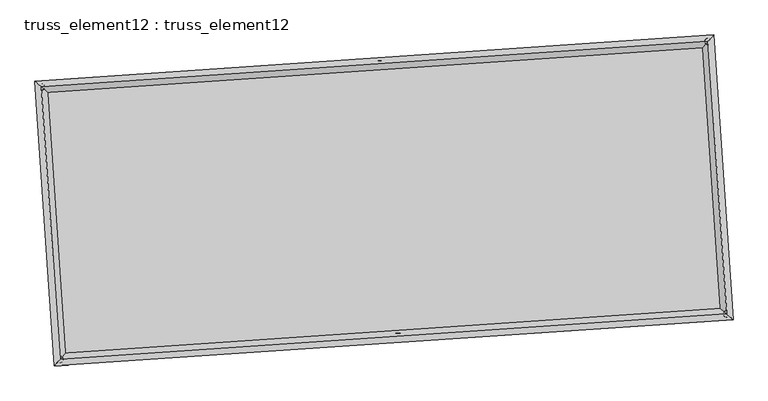
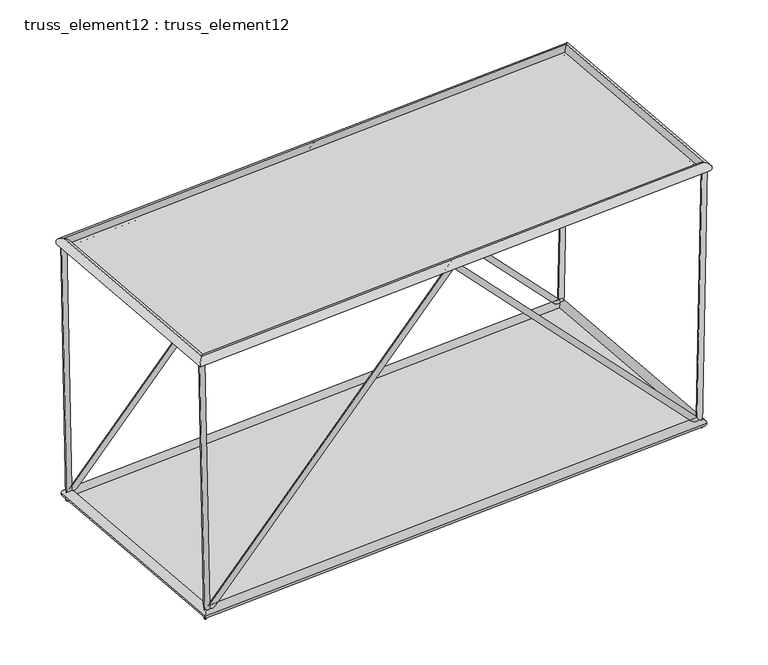
"""IFC4 building model written with IfcOpenShell, lengths in millimetres: plate geometry, truss_element12 : truss_element12."""

import ifcopenshell
import ifcopenshell.guid

model = None  # the IFC model being written
_history = None  # IfcOwnerHistory: only IFC2X3 demands one
_inside = {}  # id of a spatial element -> (the spatial element, [elements in it])
_under = {}  # id of a project, library or spatial element -> (it, [spatial elements below it])
_declared = {}  # id of a project -> (the project, [libraries it declares])
_typed = {}  # id of a type object -> (the type object, [elements of that type])
_made_of = {}  # id of a material, layer set ... -> (it, [elements and type objects made of it])


def new_model(schema):
    """Start an empty IFC model of exactly this schema.

    Asked for "IFC4X3", IfcOpenShell would pick the latest addendum, in which some entities
    have other attributes; the version numbers below select the first issue.
    IFC2X3 requires an IfcOwnerHistory on every rooted entity: one is made here for all.
    """
    global model, _history
    if schema == "IFC4X3":
        model = ifcopenshell.file(schema_version=(4, 3, 0, 0))
    else:
        model = ifcopenshell.file(schema=schema)
    _inside.clear()
    _under.clear()
    _declared.clear()
    _typed.clear()
    _made_of.clear()
    _history = None
    if model.schema == "IFC2X3":
        org = make("IfcOrganization", Name="unknown")
        user = make(
            "IfcPersonAndOrganization",
            ThePerson=make("IfcPerson", FamilyName="unknown"),
            TheOrganization=org,
        )
        app = make(
            "IfcApplication",
            ApplicationDeveloper=org,
            Version="unknown",
            ApplicationFullName="unknown",
            ApplicationIdentifier="unknown",
        )
        _history = make(
            "IfcOwnerHistory",
            OwningUser=user,
            OwningApplication=app,
            ChangeAction="ADDED",
            CreationDate=0,
        )
    return model


def make(cls, **values):
    """One entity of the class cls with the attributes given. An attribute that is None is left unset."""
    return model.create_entity(
        cls, **{name: value for name, value in values.items() if value is not None}
    )


def rooted(cls, **values):
    """An entity with a GlobalId (a new one), such as an element, a storey or a relation."""
    return make(cls, GlobalId=ifcopenshell.guid.new(), OwnerHistory=_history, **values)


def si_unit(unit_type, name, prefix=None):
    """IfcSIUnit, for example si_unit("LENGTHUNIT", "METRE", prefix="MILLI")."""
    return make("IfcSIUnit", UnitType=unit_type, Prefix=prefix, Name=name)


def assignment(units):
    """IfcUnitAssignment: the units of a project."""
    return None if units is None else make("IfcUnitAssignment", Units=units)


def point(xyz):
    """IfcCartesianPoint."""
    return None if xyz is None else make("IfcCartesianPoint", Coordinates=xyz)


def direction(xyz):
    """IfcDirection."""
    return None if xyz is None else make("IfcDirection", DirectionRatios=xyz)


def frame(location, z_axis=None, x_axis=None):
    """IfcAxis2Placement3D, a coordinate frame: its origin and axes. An axis left out is left unset."""
    return make(
        "IfcAxis2Placement3D",
        Location=point(location),
        Axis=direction(z_axis),
        RefDirection=direction(x_axis),
    )


def origin():
    """The frame at (0, 0, 0) with its axes left unset."""
    return frame((0.0, 0.0, 0.0))


def origin_with_axes():
    """The frame at (0, 0, 0) with the z axis (0, 0, 1) and the x axis (1, 0, 0) written out."""
    return frame((0.0, 0.0, 0.0), z_axis=(0.0, 0.0, 1.0), x_axis=(1.0, 0.0, 0.0))


def place(relative_to, where):
    """IfcLocalPlacement: puts the frame where relative to a parent placement (None: the world)."""
    return make(
        "IfcLocalPlacement", PlacementRelTo=relative_to, RelativePlacement=where
    )


def context(
    kind, dimensions, precision=None, world=None, true_north=None, identifier=None
):
    """IfcGeometricRepresentationContext, for example the 3D "Model" context."""
    return make(
        "IfcGeometricRepresentationContext",
        ContextIdentifier=identifier,
        ContextType=kind,
        CoordinateSpaceDimension=dimensions,
        Precision=precision,
        WorldCoordinateSystem=world,
        TrueNorth=true_north,
    )


def project(units=None, contexts=None):
    """IfcProject with its units and contexts."""
    return rooted(
        "IfcProject",
        Name="project",
        RepresentationContexts=contexts,
        UnitsInContext=assignment(units),
    )


def spatial(cls, under=None, at=None, **own):
    """A site, building, storey or space (cls), placed at a placement, below another one or the project."""
    s = rooted(cls, ObjectPlacement=at, **own)
    if under is not None:
        _under.setdefault(under.id(), (under, []))[1].append(s)
    return s


def polyline(points):
    """IfcPolyline through the points."""
    return make("IfcPolyline", Points=[point(p) for p in points])


def circle_curve(where, radius):
    """IfcCircle in the frame where."""
    return make("IfcCircle", Position=where, Radius=radius)


def ellipse_curve(where, semi_axis1, semi_axis2):
    """IfcEllipse in the frame where."""
    return make(
        "IfcEllipse", Position=where, SemiAxis1=semi_axis1, SemiAxis2=semi_axis2
    )


def outline(outer, holes=None, kind="AREA"):
    """IfcArbitraryClosedProfileDef: a profile drawn as a closed curve; with holes, ...WithVoids."""
    if holes is None:
        return make("IfcArbitraryClosedProfileDef", ProfileType=kind, OuterCurve=outer)
    return make(
        "IfcArbitraryProfileDefWithVoids",
        ProfileType=kind,
        OuterCurve=outer,
        InnerCurves=holes,
    )


def extrude(swept, where, along, depth):
    """IfcExtrudedAreaSolid: the profile swept, set in the frame where, extruded along a direction by depth."""
    return make(
        "IfcExtrudedAreaSolid",
        SweptArea=swept,
        Position=where,
        ExtrudedDirection=direction(along),
        Depth=depth,
    )


def shape(context_of_items, identifier, shape_type, items):
    """IfcShapeRepresentation: the items that make up one representation, for example the "Body"."""
    return make(
        "IfcShapeRepresentation",
        ContextOfItems=context_of_items,
        RepresentationIdentifier=identifier,
        RepresentationType=shape_type,
        Items=items,
    )


def source(mapping_origin, context_of_items, identifier, shape_type, items):
    """IfcRepresentationMap: a shape defined once, which mapped items show again and again."""
    return make(
        "IfcRepresentationMap",
        MappingOrigin=mapping_origin,
        MappedRepresentation=shape(context_of_items, identifier, shape_type, items),
    )


def transform(
    local_origin,
    x_axis=None,
    y_axis=None,
    z_axis=None,
    scale=None,
    scale2=None,
    scale3=None,
    uniform=True,
):
    """IfcCartesianTransformationOperator3D, or its non-uniform kind. x_axis, y_axis, z_axis: its Axis1, 2, 3."""
    if uniform:
        return make(
            "IfcCartesianTransformationOperator3D",
            Axis1=direction(x_axis),
            Axis2=direction(y_axis),
            LocalOrigin=point(local_origin),
            Scale=scale,
            Axis3=direction(z_axis),
        )
    return make(
        "IfcCartesianTransformationOperator3DnonUniform",
        Axis1=direction(x_axis),
        Axis2=direction(y_axis),
        LocalOrigin=point(local_origin),
        Scale=scale,
        Axis3=direction(z_axis),
        Scale2=scale2,
        Scale3=scale3,
    )


def mapped(mapping_source, mapping_target):
    """IfcMappedItem: shows the shape of a source again, moved by a transform."""
    return make(
        "IfcMappedItem", MappingSource=mapping_source, MappingTarget=mapping_target
    )


def made_of(thing, what):
    """Note that an element or type object is made of a material, layer set ...; save() writes the relation."""
    if what is not None:
        _made_of.setdefault(what.id(), (what, []))[1].append(thing)
    return thing


def element(
    cls,
    number,
    at=None,
    inside=None,
    cuts=None,
    type_object=None,
    material=None,
    context=None,
    identifier="Body",
    shape_type=None,
    held_by="IfcProductDefinitionShape",
    body=None,
    shapes=None,
    **own,
):
    """One element of the class cls, such as IfcWall. Its Tag is "e" and its number.

    at: its placement. inside: the storey or other place that contains it. cuts: it is an
    opening in that element (IfcRelVoidsElement). A single representation is given by context,
    identifier, shape_type and body (its items); several are given by shapes. held_by: the class
    of the entity that holds the representations. save() writes the other relations.
    """
    e = rooted(cls, Tag="e%d" % number, ObjectPlacement=at, **own)
    if body is not None:
        shapes = [shape(context, identifier, shape_type, body)]
    if shapes is not None:
        e.Representation = make(held_by, Representations=shapes)
    if inside is not None:
        _inside.setdefault(inside.id(), (inside, []))[1].append(e)
    if cuts is not None:
        rooted(
            "IfcRelVoidsElement", RelatingBuildingElement=cuts, RelatedOpeningElement=e
        )
    if type_object is not None:
        _typed.setdefault(type_object.id(), (type_object, []))[1].append(e)
    return made_of(e, material)


def aggregate(whole, parts):
    """IfcRelAggregates: a whole, such as a stair, and the parts it consists of."""
    return rooted("IfcRelAggregates", RelatingObject=whole, RelatedObjects=parts)


def save(model, path):
    """Write the relations noted so far, then the file.

    IfcRelAggregates (storeys below a building ...), IfcRelContainedInSpatialStructure (elements
    in a storey), IfcRelDefinesByType, IfcRelAssociatesMaterial and IfcRelDeclares: one each for
    every whole, place, type object, material and project.
    """
    for whole, parts in _under.values():
        aggregate(whole, parts)
    for where, things in _inside.values():
        rooted(
            "IfcRelContainedInSpatialStructure",
            RelatedElements=things,
            RelatingStructure=where,
        )
    for kind, things in _typed.values():
        rooted("IfcRelDefinesByType", RelatedObjects=things, RelatingType=kind)
    for what, things in _made_of.values():
        rooted("IfcRelAssociatesMaterial", RelatedObjects=things, RelatingMaterial=what)
    for by, libraries in _declared.values():
        rooted("IfcRelDeclares", RelatingContext=by, RelatedDefinitions=libraries)
    model.write(path)


def plane_surface(at):
    """IfcPlane: the flat surface through the origin of the frame at, square to its z axis."""
    return make("IfcPlane", Position=at)


def cylinder_surface(at, radius):
    """IfcCylindricalSurface: all points at the distance radius from the z axis of the frame at."""
    return make("IfcCylindricalSurface", Position=at, Radius=radius)


def advanced_brep(points, edges, surfaces, faces):
    """IfcAdvancedBrep: a solid bounded by faces that lie on surfaces and meet in shared edges.

    An edge is (start, end): straight between two places in points (the first is 0);
    or (start, end, curve); or (start, end, curve, False) where it runs against its curve.
    A face is (place in surfaces, loops), or (place, loops, False) where it looks against
    its surface's normal. A loop lists edges by number (the first is 1), with a minus sign
    where the edge is run from its end to its start. The first loop is the outer one.
    """
    corners = [point(p) for p in points]
    vertices = [make("IfcVertexPoint", VertexGeometry=c) for c in corners]
    made = []
    for start, end, *more in edges:
        made.append(
            make(
                "IfcEdgeCurve",
                EdgeStart=vertices[start],
                EdgeEnd=vertices[end],
                EdgeGeometry=more[0] if more else make("IfcPolyline", Points=[corners[start], corners[end]]),
                SameSense=more[1] if len(more) > 1 else True,
            )
        )
    hull = []
    for where, loops, *sense in faces:
        bounds = []
        for j, loop in enumerate(loops):
            ring = [make("IfcOrientedEdge", EdgeElement=made[abs(k) - 1], Orientation=k > 0) for k in loop]
            bounds.append(
                make(
                    "IfcFaceOuterBound" if j == 0 else "IfcFaceBound",
                    Bound=make("IfcEdgeLoop", EdgeList=ring),
                    Orientation=True,
                )
            )
        hull.append(make("IfcAdvancedFace", Bounds=bounds, FaceSurface=surfaces[where], SameSense=sense[0] if sense else True))
    return make("IfcAdvancedBrep", Outer=make("IfcClosedShell", CfsFaces=hull))


def truss_element12_truss_element12_cebb5c17(model_context):
    return source(origin(), model_context, "Body", "SolidModel", [
        advanced_brep(
        [(-3767.1671851, 2269.2535853, 4999.9725392), (-3866.2496537, 2255.8937932, 4997.9279448), (-3667.4174306, 2276.0551419, 121.5871098), (-3761.5694522, 2263.0315382, -121.5871098), (1064.3618326, 2598.6971827, 5071.0530248), (1064.8004406, 2592.1233545, 4926.8210996), (5794.886864, 2921.2537021, 121.578348), (5889.874113, 2921.1267864, -121.578348), (5895.881521, 2928.1401439, 4999.9589337), (5995.8598643, 2928.3535519, 4997.8888311)],
        [
            (0, 1, circle_curve(frame((-3816.7084194, 2262.5736893, 4998.950242), z_axis=(-0.020442995593720103, -0.0013939301584342944, 0.9997900484050983), x_axis=(-0.13359837212382125, 0.9910346373676144, -0.001350001298501484)), 50.0)),
            (1, 0, circle_curve(frame((-3816.7084194, 2262.5736893, 4998.950242), z_axis=(-0.020442995593720103, -0.0013939301584342944, 0.9997900484050983), x_axis=(-0.13359837212382125, 0.9910346373676144, -0.001350001298501484)), 50.0)),
            (0, 2),
            (2, 3, ellipse_curve(frame((-3714.4934414, 2269.54334, 0.0), z_axis=(-0.9295196526265942, -0.06338041167761023, 0.3632852031070248), x_axis=(0.36244361517956775, 0.024713652341926906, 0.9316779814954776)), 130.7875297, 50.0)),
            (3, 1),
            (3, 2, ellipse_curve(frame((-3714.4934414, 2269.54334, 0.0), z_axis=(-0.9295196526265942, -0.06338041167761023, 0.3632852031070248), x_axis=(0.36244361517956775, 0.024713652341926906, 0.9316779814954776)), 130.7875297, 50.0)),
            (2, 4),
            (4, 5, ellipse_curve(frame((1064.5811366, 2595.4102686, 4998.9370622), z_axis=(-0.9976833938584647, -0.06802823807757291, 6.66567062485209e-05), x_axis=(-6.650228906135178e-05, -4.534538292208103e-06, -0.9999999977784416)), 72.2729929, 50.0)),
            (5, 3),
            (5, 4, ellipse_curve(frame((1064.5811366, 2595.4102686, 4998.9370622), z_axis=(-0.9976833938584647, -0.06802823807757291, 6.66567062485209e-05), x_axis=(-6.650228906135178e-05, -4.534538292208103e-06, -0.9999999977784416)), 72.2729929, 50.0)),
            (4, 6),
            (6, 7, ellipse_curve(frame((5842.3804885, 2921.1902443, 0.0), z_axis=(-0.9295901312719009, -0.06338521734851923, -0.36310398243970066), x_axis=(-0.3622628143287533, -0.024701324219198302, 0.9317486237910036)), 130.7681897, 50.0)),
            (7, 5),
            (7, 6, ellipse_curve(frame((5842.3804885, 2921.1902443, 0.0), z_axis=(-0.9295901312719009, -0.06338521734851923, -0.36310398243970066), x_axis=(-0.3622628143287533, -0.024701324219198302, 0.9317486237910036)), 130.7681897, 50.0)),
            (8, 9, circle_curve(frame((5945.8706927, 2928.2468479, 4998.9238824), z_axis=(0.020698040829792947, 0.0014113207235643172, 0.9997847764792299), x_axis=(-0.0021628361331172694, 0.999996726933573, -0.0013668438105636789)), 50.0)),
            (9, 8, circle_curve(frame((5945.8706927, 2928.2468479, 4998.9238824), z_axis=(0.020698040829792947, 0.0014113207235643172, 0.9997847764792299), x_axis=(-0.0021628361331172694, 0.999996726933573, -0.0013668438105636789)), 50.0)),
            (6, 8),
            (9, 7),
        ],
        [
            plane_surface(frame((-3816.7084194, 2312.5736407, 4999.0199531), z_axis=(-0.020442995593718667, -0.0013939301584386158, 0.9997900484050983), x_axis=(0.9997910201292846, -2.8502064444602113e-05, 0.020442975724613167))),
            cylinder_surface(frame((-3816.7084194, 2262.5736893, 4998.950242), z_axis=(-0.0204429955937201, -0.0013939301584342942, 0.9997900484050981), x_axis=(-0.13359837212382125, 0.9910346373676144, -0.001350001298501484)), 50.0),
            cylinder_surface(frame((-3714.4934414, 2269.54334, 0.0), z_axis=(-0.6902666987206841, -0.047066662236389376, -0.7220225854799657), x_axis=(-0.020420628738629147, 0.9987517974601704, -0.04558338504321424)), 50.0),
            cylinder_surface(frame((1064.5811366, 2595.4102686, 4998.9370622), z_axis=(-0.6901706602776501, -0.0470601137400352, 0.7221148145459193), x_axis=(-0.11534629536258453, 0.9922791770993238, -0.04557704291873413)), 50.0),
            plane_surface(frame((5945.8706927, 2878.2468977, 4998.9944636), z_axis=(0.02069804082979222, 0.0014113207235603308, 0.9997847764792298), x_axis=(0.999785772606216, -2.921783322129555e-05, -0.020698020207497326))),
            cylinder_surface(frame((5842.3804885, 2921.1902443, 0.0), z_axis=(-0.020698040829792947, -0.0014113207235643172, -0.9997847764792299), x_axis=(-0.0021628361331172694, 0.999996726933573, -0.0013668438105636789)), 50.0),
        ],
        [
            (0, [[1, 2]]),
            (1, [[-1, 3, 4, 5]]),
            (1, [[-2, -5, 6, -3]]),
            (2, [[-4, 7, 8, 9]]),
            (2, [[-6, -9, 10, -7]]),
            (3, [[-8, 11, 12, 13]]),
            (3, [[-10, -13, 14, -11]]),
            (4, [[15, 16]]),
            (5, [[-12, 17, -16, 18]]),
            (5, [[-14, -18, -15, -17]]),
        ],
    ),
        advanced_brep(
        [(-3495.0542322, -1721.479999, 4999.9725392), (-3594.1367008, -1734.8397911, 4997.9279448), (-3395.3044777, -1714.6784424, 121.5871098), (-3489.4564993, -1727.7020461, -121.5871098), (1336.4747855, -1392.0364016, 5071.0530248), (1336.9133936, -1398.6102298, 4926.8210996), (6066.9998169, -1069.4798822, 121.578348), (6161.9870659, -1069.6067979, -121.578348), (6167.9944739, -1062.5934404, 4999.9589337), (6267.9728172, -1062.3800324, 4997.8888311)],
        [
            (0, 1, circle_curve(frame((-3544.5954665, -1728.159895, 4998.950242), z_axis=(-0.0204429955937201, -0.001393930158434303, 0.9997900484050983), x_axis=(-0.1335983721238217, 0.9910346373676143, -0.001350001298501484)), 50.0)),
            (1, 0, circle_curve(frame((-3544.5954665, -1728.159895, 4998.950242), z_axis=(-0.0204429955937201, -0.001393930158434303, 0.9997900484050983), x_axis=(-0.1335983721238217, 0.9910346373676143, -0.001350001298501484)), 50.0)),
            (0, 2),
            (2, 3, ellipse_curve(frame((-3442.3804885, -1721.1902443, 0.0), z_axis=(-0.9295196526265942, -0.06338041167761047, 0.3632852031070248), x_axis=(0.36244361517956775, 0.024713652341926996, 0.9316779814954776)), 130.7875297, 50.0)),
            (3, 1),
            (3, 2, ellipse_curve(frame((-3442.3804885, -1721.1902443, 0.0), z_axis=(-0.9295196526265942, -0.06338041167761047, 0.3632852031070248), x_axis=(0.36244361517956775, 0.024713652341926996, 0.9316779814954776)), 130.7875297, 50.0)),
            (2, 4),
            (4, 5, ellipse_curve(frame((1336.6940895, -1395.3233157, 4998.9370622), z_axis=(-0.9976833938584648, -0.06802823807757319, 6.66567062488419e-05), x_axis=(-6.650228906135175e-05, -4.534538292198492e-06, -0.9999999977784417)), 72.2729929, 50.0)),
            (5, 3),
            (5, 4, ellipse_curve(frame((1336.6940895, -1395.3233157, 4998.9370622), z_axis=(-0.9976833938584648, -0.06802823807757319, 6.66567062488419e-05), x_axis=(-6.650228906135175e-05, -4.534538292198492e-06, -0.9999999977784417)), 72.2729929, 50.0)),
            (4, 6),
            (6, 7, ellipse_curve(frame((6114.4934414, -1069.54334, 0.0), z_axis=(-0.9295901312719014, -0.06338521734851954, -0.3631039824397004), x_axis=(-0.36226281432875257, -0.02470132421919832, 0.931748623791004)), 130.7681897, 50.0)),
            (7, 5),
            (7, 6, ellipse_curve(frame((6114.4934414, -1069.54334, 0.0), z_axis=(-0.9295901312719014, -0.06338521734851954, -0.3631039824397004), x_axis=(-0.36226281432875257, -0.02470132421919832, 0.931748623791004)), 130.7681897, 50.0)),
            (8, 9, circle_curve(frame((6217.9836456, -1062.4867364, 4998.9238824), z_axis=(0.020698040829793325, 0.0014113207235643879, 0.9997847764792299), x_axis=(-0.0021628361331172976, 0.999996726933573, -0.0013668438105637482)), 50.0)),
            (9, 8, circle_curve(frame((6217.9836456, -1062.4867364, 4998.9238824), z_axis=(0.020698040829793325, 0.0014113207235643879, 0.9997847764792299), x_axis=(-0.0021628361331172976, 0.999996726933573, -0.0013668438105637482)), 50.0)),
            (6, 8),
            (9, 7),
        ],
        [
            plane_surface(frame((-3544.5954665, -1678.1599436, 4999.0199531), z_axis=(-0.020442995593718667, -0.0013939301584386119, 0.9997900484050983), x_axis=(0.9997910201292846, -2.8502064444602113e-05, 0.020442975724613167))),
            cylinder_surface(frame((-3544.5954665, -1728.159895, 4998.950242), z_axis=(-0.020442995593720096, -0.0013939301584343028, 0.9997900484050981), x_axis=(-0.1335983721238217, 0.9910346373676143, -0.001350001298501484)), 50.0),
            cylinder_surface(frame((-3442.3804885, -1721.1902443, 0.0), z_axis=(-0.6902666987206841, -0.04706666223638955, -0.7220225854799657), x_axis=(-0.020420628738629217, 0.9987517974601704, -0.04558338504321442)), 50.0),
            cylinder_surface(frame((1336.6940895, -1395.3233157, 4998.9370622), z_axis=(-0.6901706602776495, -0.04706011374003534, 0.7221148145459199), x_axis=(-0.11534629536258498, 0.9922791770993238, -0.04557704291873424)), 50.0),
            plane_surface(frame((6217.9836456, -1112.4866866, 4998.9944636), z_axis=(0.020698040829792222, 0.0014113207235603214, 0.9997847764792299), x_axis=(0.999785772606216, -2.9217833220407372e-05, -0.020698020207497326))),
            cylinder_surface(frame((6114.4934414, -1069.54334, 0.0), z_axis=(-0.020698040829793325, -0.0014113207235643879, -0.9997847764792299), x_axis=(-0.0021628361331172976, 0.999996726933573, -0.0013668438105637482)), 50.0),
        ],
        [
            (0, [[1, 2]]),
            (1, [[-1, 3, 4, 5]]),
            (1, [[-2, -5, 6, -3]]),
            (2, [[-4, 7, 8, 9]]),
            (2, [[-6, -9, 10, -7]]),
            (3, [[-8, 11, 12, 13]]),
            (3, [[-10, -13, 14, -11]]),
            (4, [[15, 16]]),
            (5, [[-12, 17, -16, 18]]),
            (5, [[-14, -18, -15, -17]]),
        ],
    ),
        advanced_brep(
        [(-3544.602327, -1728.1674988, 4908.9502423), (-3544.5886059, -1728.1522913, 5088.9502417), (-3816.7005902, 2262.5670871, 5088.9502417), (-3816.7162486, 2262.5802914, 4908.9502423), (5945.8643159, 2928.2392771, 5088.9238821), (5945.8770694, 2928.2544187, 4908.9238827), (6217.9763001, -1062.4801013, 5088.9238821), (6217.990991, -1062.4933716, 4908.9238827)],
        [
            (0, 1, ellipse_curve(frame((-3544.5954665, -1728.159895, 4998.950242), z_axis=(-0.7535719234028931, 0.6573654662782613, 1.9048135841045667e-06), x_axis=(-0.6573654662755273, -0.7535719234052781, 1.9048135841050712e-06)), 127.2792206, 90.0)),
            (1, 2),
            (2, 3, ellipse_curve(frame((-3816.7084194, 2262.5736893, 4998.950242), z_axis=(-0.657365466275527, -0.7535719234052783, 1.904813584105534e-06), x_axis=(0.7535719234028931, -0.6573654662782611, -1.9048135841050305e-06)), 127.2792206, 90.0)),
            (3, 0),
            (1, 0, ellipse_curve(frame((-3544.5954665, -1728.159895, 4998.950242), z_axis=(-0.7535719234028931, 0.6573654662782613, 1.9048135841045667e-06), x_axis=(-0.6573654662755273, -0.7535719234052781, 1.9048135841050712e-06)), 127.2792206, 90.0)),
            (3, 2, ellipse_curve(frame((-3816.7084194, 2262.5736893, 4998.950242), z_axis=(-0.657365466275527, -0.7535719234052783, 1.904813584105534e-06), x_axis=(0.7535719234028931, -0.6573654662782611, -1.9048135841050305e-06)), 127.2792206, 90.0)),
            (2, 4),
            (4, 5, ellipse_curve(frame((5945.8706927, 2928.2468479, 4998.9238824), z_axis=(-0.7535719234028928, 0.6573654662782618, 1.9048135841054962e-06), x_axis=(-0.6573654662755274, -0.7535719234052779, 1.9048135841050684e-06)), 127.2792206, 90.0)),
            (5, 3),
            (5, 4, ellipse_curve(frame((5945.8706927, 2928.2468479, 4998.9238824), z_axis=(-0.7535719234028928, 0.6573654662782618, 1.9048135841054962e-06), x_axis=(-0.6573654662755274, -0.7535719234052779, 1.9048135841050684e-06)), 127.2792206, 90.0)),
            (4, 6),
            (6, 7, ellipse_curve(frame((6217.9836456, -1062.4867364, 4998.9238824), z_axis=(0.6573654662755276, 0.7535719234052778, -1.9048135841046055e-06), x_axis=(-0.7535719234028927, 0.6573654662782619, 1.9048135841050322e-06)), 127.2792206, 90.0)),
            (7, 5),
            (7, 6, ellipse_curve(frame((6217.9836456, -1062.4867364, 4998.9238824), z_axis=(0.6573654662755276, 0.7535719234052778, -1.9048135841046055e-06), x_axis=(-0.7535719234028927, 0.6573654662782619, 1.9048135841050322e-06)), 127.2792206, 90.0)),
            (6, 1),
            (0, 7),
        ],
        [
            cylinder_surface(frame((-3544.5954665, -1728.159895, 4998.950242), z_axis=(0.06802823822869425, -0.9976833960748771, 0.0), x_axis=(-0.9976833927370898, -0.06802823800110322, 8.179899131489945e-05)), 90.0),
            cylinder_surface(frame((-3816.7084194, 2262.5736893, 4998.950242), z_axis=(-0.9976833960712573, -0.06802823822844584, 2.6938132044341946e-06), x_axis=(-0.068028237803244, 0.9976833929678073, 7.9105178118894e-05)), 90.0),
            cylinder_surface(frame((5945.8706927, 2928.2468479, 4998.9238824), z_axis=(-0.06802823822869297, 0.9976833960748774, 0.0), x_axis=(0.9976833931622919, 0.06802823803009485, 7.641136492288858e-05)), 90.0),
            cylinder_surface(frame((6217.9836456, -1062.4867364, 4998.9238824), z_axis=(0.9976833960712573, 0.06802823822844561, -2.693813204433539e-06), x_axis=(0.06802823822844561, -0.9976833929388144, 7.910517811889402e-05)), 90.0),
        ],
        [
            (0, [[1, 2, 3, 4]]),
            (0, [[5, -4, 6, -2]]),
            (1, [[-3, 7, 8, 9]]),
            (1, [[-6, -9, 10, -7]]),
            (2, [[-8, 11, 12, 13]]),
            (2, [[-10, -13, 14, -11]]),
            (3, [[-12, 15, -1, 16]]),
            (3, [[-14, -16, -5, -15]]),
        ],
    ),
        advanced_brep(
        [(-3358.7115243, -1625.2761972, 0.0), (-3526.0494527, -1817.1042913, 0.0), (-3810.4074885, 2353.2123043, 0.0), (-3618.5793943, 2185.8743758, 0.0), (5926.0494527, 3017.1042913, 0.0), (5758.7115243, 2825.2761972, 0.0), (6210.4074885, -1153.2123043, 0.0), (6018.5793943, -985.8743758, 0.0)],
        [
            (0, 1, ellipse_curve(frame((-3442.3804885, -1721.1902443, 0.0), z_axis=(-0.7535719234054586, 0.65736546627808, 0.0), x_axis=(-0.65736546627808, -0.7535719234054588, 0.0)), 127.2792206, 90.0)),
            (1, 2),
            (2, 3, ellipse_curve(frame((-3714.4934414, 2269.54334, 0.0), z_axis=(-0.6573654662780802, -0.7535719234054584, 0.0), x_axis=(0.7535719234054583, -0.6573654662780802, 0.0)), 127.2792206, 90.0)),
            (3, 0),
            (1, 0, ellipse_curve(frame((-3442.3804885, -1721.1902443, 0.0), z_axis=(-0.7535719234054586, 0.65736546627808, 0.0), x_axis=(-0.65736546627808, -0.7535719234054588, 0.0)), 127.2792206, 90.0)),
            (3, 2, ellipse_curve(frame((-3714.4934414, 2269.54334, 0.0), z_axis=(-0.6573654662780802, -0.7535719234054584, 0.0), x_axis=(0.7535719234054583, -0.6573654662780802, 0.0)), 127.2792206, 90.0)),
            (2, 4),
            (4, 5, ellipse_curve(frame((5842.3804885, 2921.1902443, 0.0), z_axis=(-0.7535719234054581, 0.6573654662780807, 0.0), x_axis=(-0.6573654662780806, -0.753571923405458, 0.0)), 127.2792206, 90.0)),
            (5, 3),
            (5, 4, ellipse_curve(frame((5842.3804885, 2921.1902443, 0.0), z_axis=(-0.7535719234054581, 0.6573654662780807, 0.0), x_axis=(-0.6573654662780806, -0.753571923405458, 0.0)), 127.2792206, 90.0)),
            (4, 6),
            (6, 7, ellipse_curve(frame((6114.4934414, -1069.54334, 0.0), z_axis=(0.6573654662780805, 0.7535719234054582, 0.0), x_axis=(-0.7535719234054582, 0.6573654662780806, 0.0)), 127.2792206, 90.0)),
            (7, 5),
            (7, 6, ellipse_curve(frame((6114.4934414, -1069.54334, 0.0), z_axis=(0.6573654662780805, 0.7535719234054582, 0.0), x_axis=(-0.7535719234054582, 0.6573654662780806, 0.0)), 127.2792206, 90.0)),
            (6, 1),
            (0, 7),
        ],
        [
            cylinder_surface(frame((-3442.3804885, -1721.1902443, 0.0), z_axis=(0.06802823822870284, -0.9976833960748764, 0.0), x_axis=(-0.9976833960748764, -0.06802823822870284, 0.0)), 90.0),
            cylinder_surface(frame((-3714.4934414, 2269.54334, 0.0), z_axis=(-0.9976833960748765, -0.06802823822870127, 0.0), x_axis=(-0.06802823822870127, 0.9976833960748765, 0.0)), 90.0),
            cylinder_surface(frame((5842.3804885, 2921.1902443, 0.0), z_axis=(-0.06802823822870158, 0.9976833960748765, 0.0), x_axis=(0.9976833960748765, 0.06802823822870158, 0.0)), 90.0),
            cylinder_surface(frame((6114.4934414, -1069.54334, 0.0), z_axis=(0.9976833960748767, 0.06802823822870163, 0.0), x_axis=(0.06802823822870163, -0.9976833960748767, 0.0)), 90.0),
        ],
        [
            (0, [[1, 2, 3, 4]]),
            (0, [[5, -4, 6, -2]]),
            (1, [[-3, 7, 8, 9]]),
            (1, [[-6, -9, 10, -7]]),
            (2, [[-8, 11, 12, 13]]),
            (2, [[-10, -13, 14, -11]]),
            (3, [[-12, 15, -1, 16]]),
            (3, [[-14, -16, -5, -15]]),
        ],
    ),
        extrude(outline(polyline([(-3442.3804885, -1721.1902443), (-3714.4934414, 2269.54334), (5842.3804885, 2921.1902443), (6114.4934414, -1069.54334), (-3442.3804885, -1721.1902443)])), origin_with_axes(), (0.0, 0.0, 1.0), 20.0),
        extrude(outline(polyline([(-1999.9999999, 4892.6238276), (2000.0000001, 4892.6238276), (2000.0, -4892.6238276), (-2000.0, -4892.6238276), (-1999.9999999, 4892.6238276)])), frame((1200.6376131, 600.0434764, 4998.9370622), z_axis=(2.6875727061909235e-06, 1.832553664148525e-07, 0.9999999999963718), x_axis=(-0.0680282382287029, 0.9976833960748764, 0.0)), (0.0, 0.0, 1.0), 20.0),
    ])


if __name__ == "__main__":
    model = new_model("IFC4")
    model_context = context("Model", 3, world=origin())
    ifc_project = project(units=[si_unit("LENGTHUNIT", "METRE", prefix="MILLI")], contexts=[model_context])
    site = spatial("IfcSite", under=ifc_project)
    building = spatial("IfcBuilding", under=site)
    placement = place(None, origin())
    truss_element12_truss_element12_shape = truss_element12_truss_element12_cebb5c17(model_context)
    element("IfcPlate", 1, ObjectType="truss_element12 : truss_element12", at=placement, inside=building, context=model_context, shape_type="MappedRepresentation", body=[
        mapped(truss_element12_truss_element12_shape, transform((0.0, 0.0, 0.0), x_axis=(1.0, 0.0, 0.0), y_axis=(0.0, 1.0, 0.0), z_axis=(0.0, 0.0, 1.0))),
    ])
    save(model, "model.ifc")

# Revit data of these elements
# Type "truss_element12 : truss_element12"
#   steellbar1 = 90 mm
#   steelbar2 = 50 mm
#   offset1 = 5000 mm
#   M = Default Roof
# Element 1 (IfcPlate, "truss_element12 : truss_element12")
#   Materials on its faces: "Default Roof"
# Materials
#   "Default Roof": class "Miscellaneous", colour RGB 0 127 0, transparency 0, Comments = "Rendering appearance not upgraded Rendering appearance not upgraded ", Cost = 0
